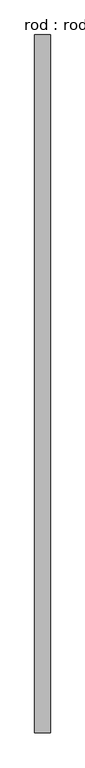
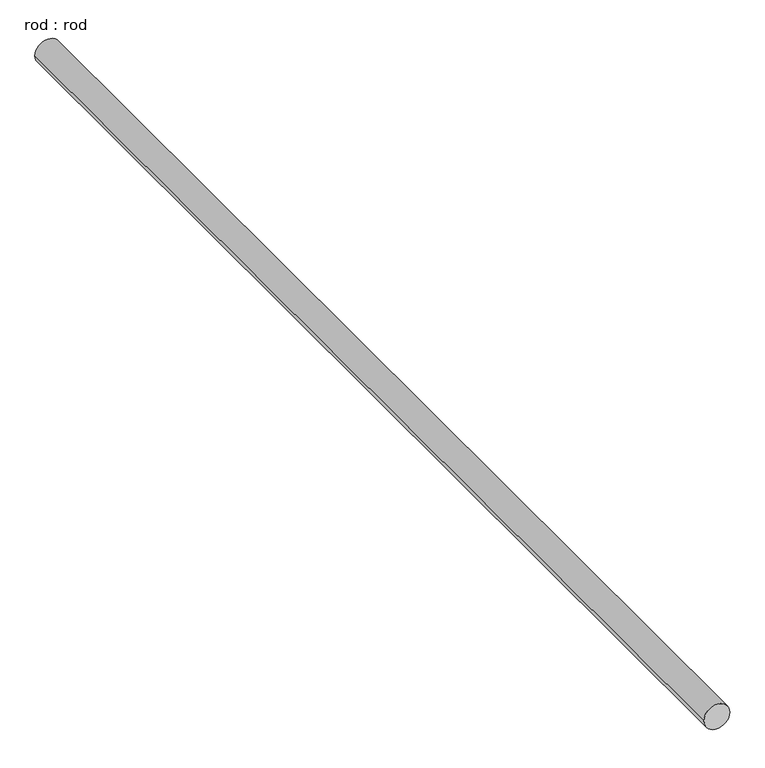
"""IFC4 building model written with IfcOpenShell, lengths in millimetres: proxy geometry, rod : rod."""

import ifcopenshell
import ifcopenshell.guid

model = None  # the IFC model being written
_history = None  # IfcOwnerHistory: only IFC2X3 demands one
_inside = {}  # id of a spatial element -> (the spatial element, [elements in it])
_under = {}  # id of a project, library or spatial element -> (it, [spatial elements below it])
_declared = {}  # id of a project -> (the project, [libraries it declares])
_typed = {}  # id of a type object -> (the type object, [elements of that type])
_made_of = {}  # id of a material, layer set ... -> (it, [elements and type objects made of it])


def new_model(schema):
    """Start an empty IFC model of exactly this schema.

    Asked for "IFC4X3", IfcOpenShell would pick the latest addendum, in which some entities
    have other attributes; the version numbers below select the first issue.
    IFC2X3 requires an IfcOwnerHistory on every rooted entity: one is made here for all.
    """
    global model, _history
    if schema == "IFC4X3":
        model = ifcopenshell.file(schema_version=(4, 3, 0, 0))
    else:
        model = ifcopenshell.file(schema=schema)
    _inside.clear()
    _under.clear()
    _declared.clear()
    _typed.clear()
    _made_of.clear()
    _history = None
    if model.schema == "IFC2X3":
        org = make("IfcOrganization", Name="unknown")
        user = make(
            "IfcPersonAndOrganization",
            ThePerson=make("IfcPerson", FamilyName="unknown"),
            TheOrganization=org,
        )
        app = make(
            "IfcApplication",
            ApplicationDeveloper=org,
            Version="unknown",
            ApplicationFullName="unknown",
            ApplicationIdentifier="unknown",
        )
        _history = make(
            "IfcOwnerHistory",
            OwningUser=user,
            OwningApplication=app,
            ChangeAction="ADDED",
            CreationDate=0,
        )
    return model


def make(cls, **values):
    """One entity of the class cls with the attributes given. An attribute that is None is left unset."""
    return model.create_entity(
        cls, **{name: value for name, value in values.items() if value is not None}
    )


def rooted(cls, **values):
    """An entity with a GlobalId (a new one), such as an element, a storey or a relation."""
    return make(cls, GlobalId=ifcopenshell.guid.new(), OwnerHistory=_history, **values)


def si_unit(unit_type, name, prefix=None):
    """IfcSIUnit, for example si_unit("LENGTHUNIT", "METRE", prefix="MILLI")."""
    return make("IfcSIUnit", UnitType=unit_type, Prefix=prefix, Name=name)


def assignment(units):
    """IfcUnitAssignment: the units of a project."""
    return None if units is None else make("IfcUnitAssignment", Units=units)


def point(xyz):
    """IfcCartesianPoint."""
    return None if xyz is None else make("IfcCartesianPoint", Coordinates=xyz)


def direction(xyz):
    """IfcDirection."""
    return None if xyz is None else make("IfcDirection", DirectionRatios=xyz)


def frame(location, z_axis=None, x_axis=None):
    """IfcAxis2Placement3D, a coordinate frame: its origin and axes. An axis left out is left unset."""
    return make(
        "IfcAxis2Placement3D",
        Location=point(location),
        Axis=direction(z_axis),
        RefDirection=direction(x_axis),
    )


def frame_2d(location, x_axis=None):
    """IfcAxis2Placement2D, a coordinate frame in the plane: its origin and x axis."""
    return make(
        "IfcAxis2Placement2D", Location=point(location), RefDirection=direction(x_axis)
    )


def origin():
    """The frame at (0, 0, 0) with its axes left unset."""
    return frame((0.0, 0.0, 0.0))


def place(relative_to, where):
    """IfcLocalPlacement: puts the frame where relative to a parent placement (None: the world)."""
    return make(
        "IfcLocalPlacement", PlacementRelTo=relative_to, RelativePlacement=where
    )


def context(
    kind, dimensions, precision=None, world=None, true_north=None, identifier=None
):
    """IfcGeometricRepresentationContext, for example the 3D "Model" context."""
    return make(
        "IfcGeometricRepresentationContext",
        ContextIdentifier=identifier,
        ContextType=kind,
        CoordinateSpaceDimension=dimensions,
        Precision=precision,
        WorldCoordinateSystem=world,
        TrueNorth=true_north,
    )


def project(units=None, contexts=None):
    """IfcProject with its units and contexts."""
    return rooted(
        "IfcProject",
        Name="project",
        RepresentationContexts=contexts,
        UnitsInContext=assignment(units),
    )


def spatial(cls, under=None, at=None, **own):
    """A site, building, storey or space (cls), placed at a placement, below another one or the project."""
    s = rooted(cls, ObjectPlacement=at, **own)
    if under is not None:
        _under.setdefault(under.id(), (under, []))[1].append(s)
    return s


def circle_curve(where, radius):
    """IfcCircle in the frame where."""
    return make("IfcCircle", Position=where, Radius=radius)


def trimmed(basis, trim1, trim2, sense, master):
    """IfcTrimmedCurve: the piece of a basis curve between two trims."""
    return make(
        "IfcTrimmedCurve",
        BasisCurve=basis,
        Trim1=trim1,
        Trim2=trim2,
        SenseAgreement=sense,
        MasterRepresentation=master,
    )


def segment(curve, same_sense, transition):
    """IfcCompositeCurveSegment."""
    return make(
        "IfcCompositeCurveSegment",
        Transition=transition,
        SameSense=same_sense,
        ParentCurve=curve,
    )


def composite_curve(segments, self_intersect=None):
    """IfcCompositeCurve: segments joined end to end."""
    return make("IfcCompositeCurve", Segments=segments, SelfIntersect=self_intersect)


def outline(outer, holes=None, kind="AREA"):
    """IfcArbitraryClosedProfileDef: a profile drawn as a closed curve; with holes, ...WithVoids."""
    if holes is None:
        return make("IfcArbitraryClosedProfileDef", ProfileType=kind, OuterCurve=outer)
    return make(
        "IfcArbitraryProfileDefWithVoids",
        ProfileType=kind,
        OuterCurve=outer,
        InnerCurves=holes,
    )


def extrude(swept, where, along, depth):
    """IfcExtrudedAreaSolid: the profile swept, set in the frame where, extruded along a direction by depth."""
    return make(
        "IfcExtrudedAreaSolid",
        SweptArea=swept,
        Position=where,
        ExtrudedDirection=direction(along),
        Depth=depth,
    )


def shape(context_of_items, identifier, shape_type, items):
    """IfcShapeRepresentation: the items that make up one representation, for example the "Body"."""
    return make(
        "IfcShapeRepresentation",
        ContextOfItems=context_of_items,
        RepresentationIdentifier=identifier,
        RepresentationType=shape_type,
        Items=items,
    )


def source(mapping_origin, context_of_items, identifier, shape_type, items):
    """IfcRepresentationMap: a shape defined once, which mapped items show again and again."""
    return make(
        "IfcRepresentationMap",
        MappingOrigin=mapping_origin,
        MappedRepresentation=shape(context_of_items, identifier, shape_type, items),
    )


def transform(
    local_origin,
    x_axis=None,
    y_axis=None,
    z_axis=None,
    scale=None,
    scale2=None,
    scale3=None,
    uniform=True,
):
    """IfcCartesianTransformationOperator3D, or its non-uniform kind. x_axis, y_axis, z_axis: its Axis1, 2, 3."""
    if uniform:
        return make(
            "IfcCartesianTransformationOperator3D",
            Axis1=direction(x_axis),
            Axis2=direction(y_axis),
            LocalOrigin=point(local_origin),
            Scale=scale,
            Axis3=direction(z_axis),
        )
    return make(
        "IfcCartesianTransformationOperator3DnonUniform",
        Axis1=direction(x_axis),
        Axis2=direction(y_axis),
        LocalOrigin=point(local_origin),
        Scale=scale,
        Axis3=direction(z_axis),
        Scale2=scale2,
        Scale3=scale3,
    )


def mapped(mapping_source, mapping_target):
    """IfcMappedItem: shows the shape of a source again, moved by a transform."""
    return make(
        "IfcMappedItem", MappingSource=mapping_source, MappingTarget=mapping_target
    )


def made_of(thing, what):
    """Note that an element or type object is made of a material, layer set ...; save() writes the relation."""
    if what is not None:
        _made_of.setdefault(what.id(), (what, []))[1].append(thing)
    return thing


def element(
    cls,
    number,
    at=None,
    inside=None,
    cuts=None,
    type_object=None,
    material=None,
    context=None,
    identifier="Body",
    shape_type=None,
    held_by="IfcProductDefinitionShape",
    body=None,
    shapes=None,
    **own,
):
    """One element of the class cls, such as IfcWall. Its Tag is "e" and its number.

    at: its placement. inside: the storey or other place that contains it. cuts: it is an
    opening in that element (IfcRelVoidsElement). A single representation is given by context,
    identifier, shape_type and body (its items); several are given by shapes. held_by: the class
    of the entity that holds the representations. save() writes the other relations.
    """
    e = rooted(cls, Tag="e%d" % number, ObjectPlacement=at, **own)
    if body is not None:
        shapes = [shape(context, identifier, shape_type, body)]
    if shapes is not None:
        e.Representation = make(held_by, Representations=shapes)
    if inside is not None:
        _inside.setdefault(inside.id(), (inside, []))[1].append(e)
    if cuts is not None:
        rooted(
            "IfcRelVoidsElement", RelatingBuildingElement=cuts, RelatedOpeningElement=e
        )
    if type_object is not None:
        _typed.setdefault(type_object.id(), (type_object, []))[1].append(e)
    return made_of(e, material)


def aggregate(whole, parts):
    """IfcRelAggregates: a whole, such as a stair, and the parts it consists of."""
    return rooted("IfcRelAggregates", RelatingObject=whole, RelatedObjects=parts)


def save(model, path):
    """Write the relations noted so far, then the file.

    IfcRelAggregates (storeys below a building ...), IfcRelContainedInSpatialStructure (elements
    in a storey), IfcRelDefinesByType, IfcRelAssociatesMaterial and IfcRelDeclares: one each for
    every whole, place, type object, material and project.
    """
    for whole, parts in _under.values():
        aggregate(whole, parts)
    for where, things in _inside.values():
        rooted(
            "IfcRelContainedInSpatialStructure",
            RelatedElements=things,
            RelatingStructure=where,
        )
    for kind, things in _typed.values():
        rooted("IfcRelDefinesByType", RelatedObjects=things, RelatingType=kind)
    for what, things in _made_of.values():
        rooted("IfcRelAssociatesMaterial", RelatedObjects=things, RelatingMaterial=what)
    for by, libraries in _declared.values():
        rooted("IfcRelDeclares", RelatingContext=by, RelatedDefinitions=libraries)
    model.write(path)


def rod_rod_cc858682(model_context):
    return source(origin(), model_context, "Body", "SweptSolid", [
        extrude(outline(composite_curve([segment(trimmed(circle_curve(frame_2d((0.0108462, 0.0)), 200.0), [point((0.0108462, 200.0))], [point((0.0108462, -200.0))], False, "CARTESIAN"), True, "CONTINUOUS"), segment(trimmed(circle_curve(frame_2d((0.0108462, 0.0)), 200.0), [point((0.0108462, -200.0))], [point((0.0108462, 200.0))], False, "CARTESIAN"), True, "CONTINUOUS")], self_intersect=False)), frame((0.0, -4835.8428132, 0.0), z_axis=(0.0, 1.0, 0.0), x_axis=(0.0, 0.0, 1.0)), (0.0, 0.0, 1.0), 17857.1428571),
    ])


if __name__ == "__main__":
    model = new_model("IFC4")
    model_context = context("Model", 3, world=origin())
    ifc_project = project(units=[si_unit("LENGTHUNIT", "METRE", prefix="MILLI")], contexts=[model_context])
    site = spatial("IfcSite", under=ifc_project)
    building = spatial("IfcBuilding", under=site)
    placement = place(None, origin())
    rod_rod_shape = rod_rod_cc858682(model_context)
    element("IfcBuildingElementProxy", 1, Name="rod : rod", ObjectType="rod : rod", at=placement, inside=building, context=model_context, shape_type="MappedRepresentation", body=[
        mapped(rod_rod_shape, transform((0.0, 0.0, 0.0), x_axis=(1.0, 0.0, 0.0), y_axis=(0.0, 1.0, 0.0), z_axis=(0.0, 0.0, 1.0))),
    ])
    save(model, "model.ifc")

# Revit data of these elements
# Type "rod : rod"
#   Default Elevation = 0
